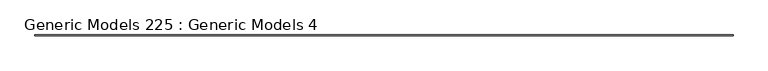
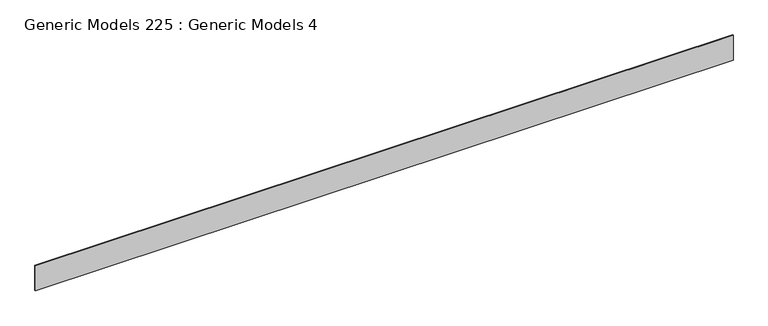
"""IFC4 building model written with IfcOpenShell, lengths in millimetres: proxy geometry, Generic Models 225 : Generic Models 4."""

from ifc_helpers import new_model, si_unit, frame, origin, place, context, project, spatial, polyline, outline, extrude, source, transform, mapped, element, save


def generic_models_225_generic_models_4_75ce27d7(model_context):
    return source(origin(), model_context, "Body", "SweptSolid", [
        extrude(outline(polyline([(-2152.1733045, -29321.7235482), (-2152.1733045, -29340.7735482), (-20795.7733045, -29340.7735482), (-20795.7733045, -29321.7235482), (-2152.1733045, -29321.7235482)])), frame((0.0, 0.0, 126371.3358061), z_axis=(0.0, 0.0, 1.0), x_axis=(1.0, 0.0, 0.0)), (0.0, 0.0, 1.0), 698.058176),
    ])


if __name__ == "__main__":
    model = new_model("IFC4")
    model_context = context("Model", 3, world=origin())
    ifc_project = project(units=[si_unit("LENGTHUNIT", "METRE", prefix="MILLI")], contexts=[model_context])
    site = spatial("IfcSite", under=ifc_project)
    building = spatial("IfcBuilding", under=site)
    placement = place(None, origin())
    generic_models_225_generic_models_4_shape = generic_models_225_generic_models_4_75ce27d7(model_context)
    element("IfcBuildingElementProxy", 1, Name="Generic Models 225 : Generic Models 4", ObjectType="Generic Models 225 : Generic Models 4", at=placement, inside=building, context=model_context, shape_type="MappedRepresentation", body=[
        mapped(generic_models_225_generic_models_4_shape, transform((0.0, 0.0, 0.0), x_axis=(1.0, 0.0, 0.0), y_axis=(0.0, 1.0, 0.0), z_axis=(0.0, 0.0, 1.0))),
    ])
    save(model, "model.ifc")

# Revit data of these elements
# Element 1 (IfcBuildingElementProxy, "Generic Models 225 : Generic Models 4")
#   Materials on its faces: "_CDX PLYWOOD - SEE STRUCT DWGs"
# Materials
#   "_CDX PLYWOOD - SEE STRUCT DWGs": class "Generic", colour RGB 98 75 74, transparency 0, Cost = 0
